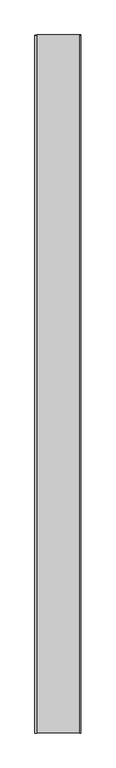
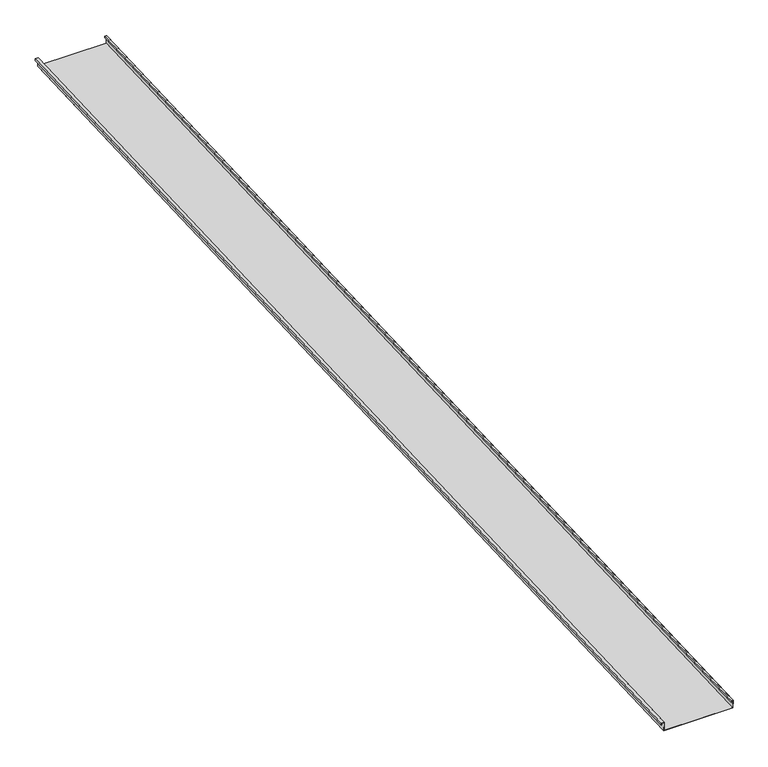
"""IFC4 building model written with IfcOpenShell, lengths in millimetres: proxy geometry, Generic Models 2:Generic Models 2:310765:Generic Models 2:310765 : Generic Models 2:Generic Models 2:310765:113 : Generic Models 2:Generic Models 2:310765:Generic Models 2:310765 : Generic Models 2:Generic Models 2:310765:300385."""

import ifcopenshell
import ifcopenshell.guid

model = None  # the IFC model being written
_history = None  # IfcOwnerHistory: only IFC2X3 demands one
_inside = {}  # id of a spatial element -> (the spatial element, [elements in it])
_under = {}  # id of a project, library or spatial element -> (it, [spatial elements below it])
_declared = {}  # id of a project -> (the project, [libraries it declares])
_typed = {}  # id of a type object -> (the type object, [elements of that type])
_made_of = {}  # id of a material, layer set ... -> (it, [elements and type objects made of it])


def new_model(schema):
    """Start an empty IFC model of exactly this schema.

    Asked for "IFC4X3", IfcOpenShell would pick the latest addendum, in which some entities
    have other attributes; the version numbers below select the first issue.
    IFC2X3 requires an IfcOwnerHistory on every rooted entity: one is made here for all.
    """
    global model, _history
    if schema == "IFC4X3":
        model = ifcopenshell.file(schema_version=(4, 3, 0, 0))
    else:
        model = ifcopenshell.file(schema=schema)
    _inside.clear()
    _under.clear()
    _declared.clear()
    _typed.clear()
    _made_of.clear()
    _history = None
    if model.schema == "IFC2X3":
        org = make("IfcOrganization", Name="unknown")
        user = make(
            "IfcPersonAndOrganization",
            ThePerson=make("IfcPerson", FamilyName="unknown"),
            TheOrganization=org,
        )
        app = make(
            "IfcApplication",
            ApplicationDeveloper=org,
            Version="unknown",
            ApplicationFullName="unknown",
            ApplicationIdentifier="unknown",
        )
        _history = make(
            "IfcOwnerHistory",
            OwningUser=user,
            OwningApplication=app,
            ChangeAction="ADDED",
            CreationDate=0,
        )
    return model


def make(cls, **values):
    """One entity of the class cls with the attributes given. An attribute that is None is left unset."""
    return model.create_entity(
        cls, **{name: value for name, value in values.items() if value is not None}
    )


def rooted(cls, **values):
    """An entity with a GlobalId (a new one), such as an element, a storey or a relation."""
    return make(cls, GlobalId=ifcopenshell.guid.new(), OwnerHistory=_history, **values)


def si_unit(unit_type, name, prefix=None):
    """IfcSIUnit, for example si_unit("LENGTHUNIT", "METRE", prefix="MILLI")."""
    return make("IfcSIUnit", UnitType=unit_type, Prefix=prefix, Name=name)


def assignment(units):
    """IfcUnitAssignment: the units of a project."""
    return None if units is None else make("IfcUnitAssignment", Units=units)


def point(xyz):
    """IfcCartesianPoint."""
    return None if xyz is None else make("IfcCartesianPoint", Coordinates=xyz)


def direction(xyz):
    """IfcDirection."""
    return None if xyz is None else make("IfcDirection", DirectionRatios=xyz)


def frame(location, z_axis=None, x_axis=None):
    """IfcAxis2Placement3D, a coordinate frame: its origin and axes. An axis left out is left unset."""
    return make(
        "IfcAxis2Placement3D",
        Location=point(location),
        Axis=direction(z_axis),
        RefDirection=direction(x_axis),
    )


def origin():
    """The frame at (0, 0, 0) with its axes left unset."""
    return frame((0.0, 0.0, 0.0))


def place(relative_to, where):
    """IfcLocalPlacement: puts the frame where relative to a parent placement (None: the world)."""
    return make(
        "IfcLocalPlacement", PlacementRelTo=relative_to, RelativePlacement=where
    )


def context(
    kind, dimensions, precision=None, world=None, true_north=None, identifier=None
):
    """IfcGeometricRepresentationContext, for example the 3D "Model" context."""
    return make(
        "IfcGeometricRepresentationContext",
        ContextIdentifier=identifier,
        ContextType=kind,
        CoordinateSpaceDimension=dimensions,
        Precision=precision,
        WorldCoordinateSystem=world,
        TrueNorth=true_north,
    )


def project(units=None, contexts=None):
    """IfcProject with its units and contexts."""
    return rooted(
        "IfcProject",
        Name="project",
        RepresentationContexts=contexts,
        UnitsInContext=assignment(units),
    )


def spatial(cls, under=None, at=None, **own):
    """A site, building, storey or space (cls), placed at a placement, below another one or the project."""
    s = rooted(cls, ObjectPlacement=at, **own)
    if under is not None:
        _under.setdefault(under.id(), (under, []))[1].append(s)
    return s


def polyline(points):
    """IfcPolyline through the points."""
    return make("IfcPolyline", Points=[point(p) for p in points])


def outline(outer, holes=None, kind="AREA"):
    """IfcArbitraryClosedProfileDef: a profile drawn as a closed curve; with holes, ...WithVoids."""
    if holes is None:
        return make("IfcArbitraryClosedProfileDef", ProfileType=kind, OuterCurve=outer)
    return make(
        "IfcArbitraryProfileDefWithVoids",
        ProfileType=kind,
        OuterCurve=outer,
        InnerCurves=holes,
    )


def extrude(swept, where, along, depth):
    """IfcExtrudedAreaSolid: the profile swept, set in the frame where, extruded along a direction by depth."""
    return make(
        "IfcExtrudedAreaSolid",
        SweptArea=swept,
        Position=where,
        ExtrudedDirection=direction(along),
        Depth=depth,
    )


def shape(context_of_items, identifier, shape_type, items):
    """IfcShapeRepresentation: the items that make up one representation, for example the "Body"."""
    return make(
        "IfcShapeRepresentation",
        ContextOfItems=context_of_items,
        RepresentationIdentifier=identifier,
        RepresentationType=shape_type,
        Items=items,
    )


def source(mapping_origin, context_of_items, identifier, shape_type, items):
    """IfcRepresentationMap: a shape defined once, which mapped items show again and again."""
    return make(
        "IfcRepresentationMap",
        MappingOrigin=mapping_origin,
        MappedRepresentation=shape(context_of_items, identifier, shape_type, items),
    )


def transform(
    local_origin,
    x_axis=None,
    y_axis=None,
    z_axis=None,
    scale=None,
    scale2=None,
    scale3=None,
    uniform=True,
):
    """IfcCartesianTransformationOperator3D, or its non-uniform kind. x_axis, y_axis, z_axis: its Axis1, 2, 3."""
    if uniform:
        return make(
            "IfcCartesianTransformationOperator3D",
            Axis1=direction(x_axis),
            Axis2=direction(y_axis),
            LocalOrigin=point(local_origin),
            Scale=scale,
            Axis3=direction(z_axis),
        )
    return make(
        "IfcCartesianTransformationOperator3DnonUniform",
        Axis1=direction(x_axis),
        Axis2=direction(y_axis),
        LocalOrigin=point(local_origin),
        Scale=scale,
        Axis3=direction(z_axis),
        Scale2=scale2,
        Scale3=scale3,
    )


def mapped(mapping_source, mapping_target):
    """IfcMappedItem: shows the shape of a source again, moved by a transform."""
    return make(
        "IfcMappedItem", MappingSource=mapping_source, MappingTarget=mapping_target
    )


def made_of(thing, what):
    """Note that an element or type object is made of a material, layer set ...; save() writes the relation."""
    if what is not None:
        _made_of.setdefault(what.id(), (what, []))[1].append(thing)
    return thing


def element(
    cls,
    number,
    at=None,
    inside=None,
    cuts=None,
    type_object=None,
    material=None,
    context=None,
    identifier="Body",
    shape_type=None,
    held_by="IfcProductDefinitionShape",
    body=None,
    shapes=None,
    **own,
):
    """One element of the class cls, such as IfcWall. Its Tag is "e" and its number.

    at: its placement. inside: the storey or other place that contains it. cuts: it is an
    opening in that element (IfcRelVoidsElement). A single representation is given by context,
    identifier, shape_type and body (its items); several are given by shapes. held_by: the class
    of the entity that holds the representations. save() writes the other relations.
    """
    e = rooted(cls, Tag="e%d" % number, ObjectPlacement=at, **own)
    if body is not None:
        shapes = [shape(context, identifier, shape_type, body)]
    if shapes is not None:
        e.Representation = make(held_by, Representations=shapes)
    if inside is not None:
        _inside.setdefault(inside.id(), (inside, []))[1].append(e)
    if cuts is not None:
        rooted(
            "IfcRelVoidsElement", RelatingBuildingElement=cuts, RelatedOpeningElement=e
        )
    if type_object is not None:
        _typed.setdefault(type_object.id(), (type_object, []))[1].append(e)
    return made_of(e, material)


def aggregate(whole, parts):
    """IfcRelAggregates: a whole, such as a stair, and the parts it consists of."""
    return rooted("IfcRelAggregates", RelatingObject=whole, RelatedObjects=parts)


def save(model, path):
    """Write the relations noted so far, then the file.

    IfcRelAggregates (storeys below a building ...), IfcRelContainedInSpatialStructure (elements
    in a storey), IfcRelDefinesByType, IfcRelAssociatesMaterial and IfcRelDeclares: one each for
    every whole, place, type object, material and project.
    """
    for whole, parts in _under.values():
        aggregate(whole, parts)
    for where, things in _inside.values():
        rooted(
            "IfcRelContainedInSpatialStructure",
            RelatedElements=things,
            RelatingStructure=where,
        )
    for kind, things in _typed.values():
        rooted("IfcRelDefinesByType", RelatedObjects=things, RelatingType=kind)
    for what, things in _made_of.values():
        rooted("IfcRelAssociatesMaterial", RelatedObjects=things, RelatingMaterial=what)
    for by, libraries in _declared.values():
        rooted("IfcRelDeclares", RelatingContext=by, RelatedDefinitions=libraries)
    model.write(path)


def generic_models_9320bea5(model_context):
    return source(origin(), model_context, "Body", "SweptSolid", [
        extrude(outline(polyline([(1.5875, 0.0), (1.5875, 50.8), (407.9875, 50.8), (407.9875, 1.5875), (396.875, 1.5875), (396.875, 11.1125), (398.4625, 11.1125), (398.4625, 3.175), (406.4, 3.175), (406.4, 49.2125), (3.175, 49.2125), (3.175, -1.5874999), (-14.2875, -1.5874999), (-14.2875, 9.525), (-12.7, 9.525), (-12.7, 0.0), (1.5875, 0.0)])), frame((607834.2929739, -581354.4345603, 3902.6697972), z_axis=(0.0, 0.9991330730923568, 0.041630544712067834), x_axis=(1.0, 0.0, 0.0)), (0.0, 0.0, 1.0), 6400.8),
    ])


if __name__ == "__main__":
    model = new_model("IFC4")
    model_context = context("Model", 3, world=origin())
    ifc_project = project(units=[si_unit("LENGTHUNIT", "METRE", prefix="MILLI")], contexts=[model_context])
    site = spatial("IfcSite", under=ifc_project)
    building = spatial("IfcBuilding", under=site)
    placement = place(None, origin())
    generic_models_shape = generic_models_9320bea5(model_context)
    element("IfcBuildingElementProxy", 1, Name="Generic Models 2:Generic Models 2:310765:Generic Models 2:310765 : Generic Models 2:Generic Models 2:310765:113 : Generic Models 2:Generic Models 2:310765:Generic Models 2:310765 : Generic Models 2:Generic Models 2:310765:300385", ObjectType="Generic Models 2:Generic Models 2:310765:Generic Models 2:310765 : Generic Models 2:Generic Models 2:310765:113 : Generic Models 2:Generic Models 2:310765:Generic Models 2:310765 : Generic Models 2:Generic Models 2:310765:300385", at=placement, inside=building, context=model_context, shape_type="MappedRepresentation", body=[
        mapped(generic_models_shape, transform((0.0, 0.0, 0.0), x_axis=(1.0, 0.0, 0.0), y_axis=(0.0, 1.0, 0.0), z_axis=(0.0, 0.0, 1.0))),
    ])
    save(model, "model.ifc")

# Revit data of these elements
# Type "Generic Models 2:Generic Models 2:310765:Generic Models 2:310765 : Generic Models 2:Generic Models 2:310765:113 : Generic Models 2:Generic Models 2:310765:Generic Models 2:310765 : Generic Models 2:Generic Models 2:310765:300385"
#   NameOverride = "Generic Models 2:Generic Models 2:310765:Generic Models 2:310765 : Generic Models 2:Generic Models 2:310765:300385"
#   ObjectTypeOverride = "Generic Models 2:310765 : Generic Models 2:Generic Models 2:310765"
#   Reference = "Generic Models 2"
#   Tag = "300385"
# Element 1 (IfcBuildingElementProxy, "Generic Models 2:Generic Models 2:310765:Generic Models 2:310765 : Generic Models 2:Generic Models 2:310765:113 : Generic Models 2:Generic Models 2:310765:Generic Models 2:310765 : Generic Models 2:Generic Models 2:310765:300385")
#   Materials on its faces: "THERMAL BROKEN ALUMINUM STOREFRONT FOR POLYCARBONATE"
# Materials
#   "THERMAL BROKEN ALUMINUM STOREFRONT FOR POLYCARBONATE": class "Unassigned", colour RGB 244 244 244, transparency 0, Keynote = "M07611300.01", Cost = 0
